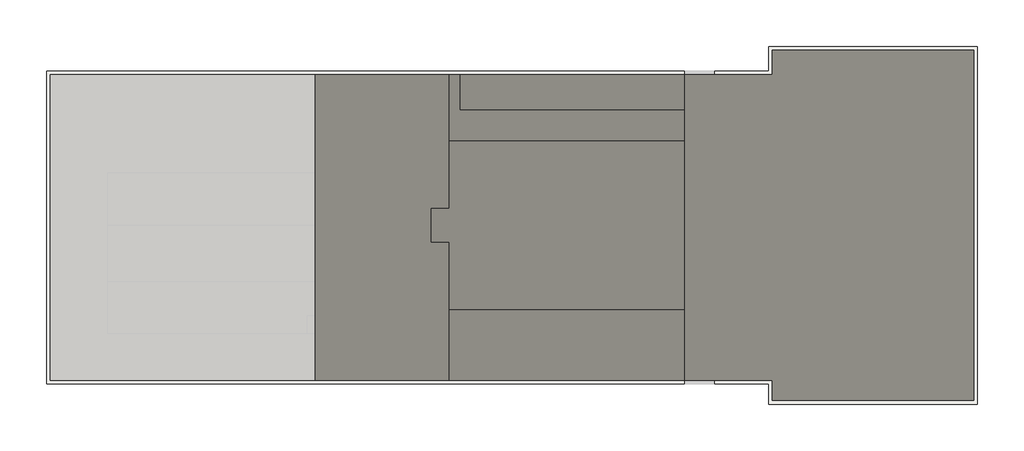
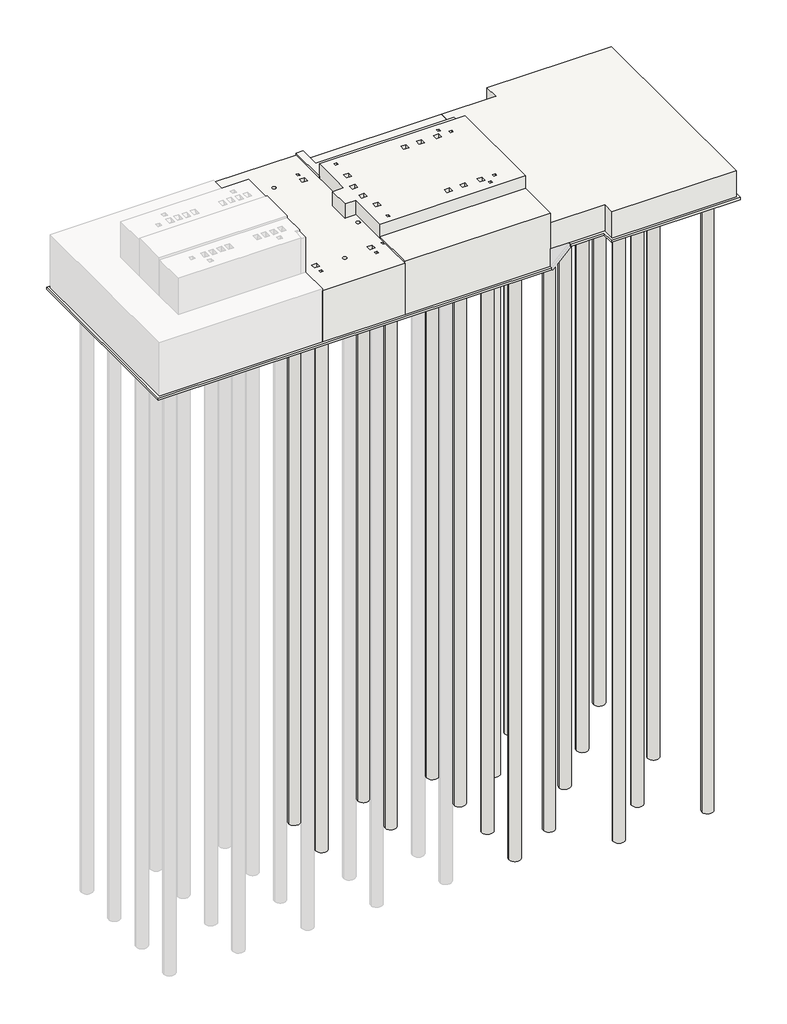
# One storey, part 2 of 2: 25 slabs.
"""IFC4 building model written with IfcOpenShell, lengths in millimetres."""

import ifcopenshell
import ifcopenshell.guid

model = None  # the IFC model being written
_history = None  # IfcOwnerHistory: only IFC2X3 demands one
_inside = {}  # id of a spatial element -> (the spatial element, [elements in it])
_under = {}  # id of a project, library or spatial element -> (it, [spatial elements below it])
_declared = {}  # id of a project -> (the project, [libraries it declares])
_typed = {}  # id of a type object -> (the type object, [elements of that type])
_made_of = {}  # id of a material, layer set ... -> (it, [elements and type objects made of it])


def new_model(schema):
    """Start an empty IFC model of exactly this schema.

    Asked for "IFC4X3", IfcOpenShell would pick the latest addendum, in which some entities
    have other attributes; the version numbers below select the first issue.
    IFC2X3 requires an IfcOwnerHistory on every rooted entity: one is made here for all.
    """
    global model, _history
    if schema == "IFC4X3":
        model = ifcopenshell.file(schema_version=(4, 3, 0, 0))
    else:
        model = ifcopenshell.file(schema=schema)
    _inside.clear()
    _under.clear()
    _declared.clear()
    _typed.clear()
    _made_of.clear()
    _history = None
    if model.schema == "IFC2X3":
        org = make("IfcOrganization", Name="unknown")
        user = make(
            "IfcPersonAndOrganization",
            ThePerson=make("IfcPerson", FamilyName="unknown"),
            TheOrganization=org,
        )
        app = make(
            "IfcApplication",
            ApplicationDeveloper=org,
            Version="unknown",
            ApplicationFullName="unknown",
            ApplicationIdentifier="unknown",
        )
        _history = make(
            "IfcOwnerHistory",
            OwningUser=user,
            OwningApplication=app,
            ChangeAction="ADDED",
            CreationDate=0,
        )
    return model


def make(cls, **values):
    """One entity of the class cls with the attributes given. An attribute that is None is left unset."""
    return model.create_entity(
        cls, **{name: value for name, value in values.items() if value is not None}
    )


def rooted(cls, **values):
    """An entity with a GlobalId (a new one), such as an element, a storey or a relation."""
    return make(cls, GlobalId=ifcopenshell.guid.new(), OwnerHistory=_history, **values)


def si_unit(unit_type, name, prefix=None):
    """IfcSIUnit, for example si_unit("LENGTHUNIT", "METRE", prefix="MILLI")."""
    return make("IfcSIUnit", UnitType=unit_type, Prefix=prefix, Name=name)


def assignment(units):
    """IfcUnitAssignment: the units of a project."""
    return None if units is None else make("IfcUnitAssignment", Units=units)


def point(xyz):
    """IfcCartesianPoint."""
    return None if xyz is None else make("IfcCartesianPoint", Coordinates=xyz)


def direction(xyz):
    """IfcDirection."""
    return None if xyz is None else make("IfcDirection", DirectionRatios=xyz)


def frame(location, z_axis=None, x_axis=None):
    """IfcAxis2Placement3D, a coordinate frame: its origin and axes. An axis left out is left unset."""
    return make(
        "IfcAxis2Placement3D",
        Location=point(location),
        Axis=direction(z_axis),
        RefDirection=direction(x_axis),
    )


def frame_2d(location, x_axis=None):
    """IfcAxis2Placement2D, a coordinate frame in the plane: its origin and x axis."""
    return make(
        "IfcAxis2Placement2D", Location=point(location), RefDirection=direction(x_axis)
    )


def origin():
    """The frame at (0, 0, 0) with its axes left unset."""
    return frame((0.0, 0.0, 0.0))


def place(relative_to, where):
    """IfcLocalPlacement: puts the frame where relative to a parent placement (None: the world)."""
    return make(
        "IfcLocalPlacement", PlacementRelTo=relative_to, RelativePlacement=where
    )


def context(
    kind, dimensions, precision=None, world=None, true_north=None, identifier=None
):
    """IfcGeometricRepresentationContext, for example the 3D "Model" context."""
    return make(
        "IfcGeometricRepresentationContext",
        ContextIdentifier=identifier,
        ContextType=kind,
        CoordinateSpaceDimension=dimensions,
        Precision=precision,
        WorldCoordinateSystem=world,
        TrueNorth=true_north,
    )


def project(units=None, contexts=None):
    """IfcProject with its units and contexts."""
    return rooted(
        "IfcProject",
        Name="project",
        RepresentationContexts=contexts,
        UnitsInContext=assignment(units),
    )


def spatial(cls, under=None, at=None, **own):
    """A site, building, storey or space (cls), placed at a placement, below another one or the project."""
    s = rooted(cls, ObjectPlacement=at, **own)
    if under is not None:
        _under.setdefault(under.id(), (under, []))[1].append(s)
    return s


def polyline(points):
    """IfcPolyline through the points."""
    return make("IfcPolyline", Points=[point(p) for p in points])


def circle_curve(where, radius):
    """IfcCircle in the frame where."""
    return make("IfcCircle", Position=where, Radius=radius)


def trimmed(basis, trim1, trim2, sense, master):
    """IfcTrimmedCurve: the piece of a basis curve between two trims."""
    return make(
        "IfcTrimmedCurve",
        BasisCurve=basis,
        Trim1=trim1,
        Trim2=trim2,
        SenseAgreement=sense,
        MasterRepresentation=master,
    )


def segment(curve, same_sense, transition):
    """IfcCompositeCurveSegment."""
    return make(
        "IfcCompositeCurveSegment",
        Transition=transition,
        SameSense=same_sense,
        ParentCurve=curve,
    )


def composite_curve(segments, self_intersect=None):
    """IfcCompositeCurve: segments joined end to end."""
    return make("IfcCompositeCurve", Segments=segments, SelfIntersect=self_intersect)


def outline(outer, holes=None, kind="AREA"):
    """IfcArbitraryClosedProfileDef: a profile drawn as a closed curve; with holes, ...WithVoids."""
    if holes is None:
        return make("IfcArbitraryClosedProfileDef", ProfileType=kind, OuterCurve=outer)
    return make(
        "IfcArbitraryProfileDefWithVoids",
        ProfileType=kind,
        OuterCurve=outer,
        InnerCurves=holes,
    )


def extrude(swept, where, along, depth):
    """IfcExtrudedAreaSolid: the profile swept, set in the frame where, extruded along a direction by depth."""
    return make(
        "IfcExtrudedAreaSolid",
        SweptArea=swept,
        Position=where,
        ExtrudedDirection=direction(along),
        Depth=depth,
    )


def faces_of(points, faces, orient=None, outer=None):
    """IfcFace entities. A face is a list of loops; a loop is a list of indices into points, from 0.

    orient and outer hold one flag for each loop. By default every Orientation is true, the
    first loop of a face is its IfcFaceOuterBound and the others are IfcFaceBound.
    """
    made = []
    for i, loops in enumerate(faces):
        bounds = []
        for j, loop in enumerate(loops):
            is_outer = j == 0 if outer is None else outer[i][j]
            bounds.append(
                make(
                    "IfcFaceOuterBound" if is_outer else "IfcFaceBound",
                    Bound=make("IfcPolyLoop", Polygon=[points[k] for k in loop]),
                    Orientation=True if orient is None else orient[i][j],
                )
            )
        made.append(make("IfcFace", Bounds=bounds))
    return made


def faceted_brep(points, faces, orient=None, outer=None, voids=None):
    """IfcFacetedBrep: a solid bounded by flat faces; with voids (closed shells), ...WithVoids."""
    shared = [point(p) for p in points]
    hull = make("IfcClosedShell", CfsFaces=faces_of(shared, faces, orient, outer))
    if voids is None:
        return make("IfcFacetedBrep", Outer=hull)
    return make(
        "IfcFacetedBrepWithVoids",
        Outer=hull,
        Voids=[
            make(cls, CfsFaces=faces_of(shared, fs, o, b)) for cls, fs, o, b in voids
        ],
    )


def shape(context_of_items, identifier, shape_type, items):
    """IfcShapeRepresentation: the items that make up one representation, for example the "Body"."""
    return make(
        "IfcShapeRepresentation",
        ContextOfItems=context_of_items,
        RepresentationIdentifier=identifier,
        RepresentationType=shape_type,
        Items=items,
    )


def made_of(thing, what):
    """Note that an element or type object is made of a material, layer set ...; save() writes the relation."""
    if what is not None:
        _made_of.setdefault(what.id(), (what, []))[1].append(thing)
    return thing


def element(
    cls,
    number,
    at=None,
    inside=None,
    cuts=None,
    type_object=None,
    material=None,
    context=None,
    identifier="Body",
    shape_type=None,
    held_by="IfcProductDefinitionShape",
    body=None,
    shapes=None,
    **own,
):
    """One element of the class cls, such as IfcWall. Its Tag is "e" and its number.

    at: its placement. inside: the storey or other place that contains it. cuts: it is an
    opening in that element (IfcRelVoidsElement). A single representation is given by context,
    identifier, shape_type and body (its items); several are given by shapes. held_by: the class
    of the entity that holds the representations. save() writes the other relations.
    """
    e = rooted(cls, Tag="e%d" % number, ObjectPlacement=at, **own)
    if body is not None:
        shapes = [shape(context, identifier, shape_type, body)]
    if shapes is not None:
        e.Representation = make(held_by, Representations=shapes)
    if inside is not None:
        _inside.setdefault(inside.id(), (inside, []))[1].append(e)
    if cuts is not None:
        rooted(
            "IfcRelVoidsElement", RelatingBuildingElement=cuts, RelatedOpeningElement=e
        )
    if type_object is not None:
        _typed.setdefault(type_object.id(), (type_object, []))[1].append(e)
    return made_of(e, material)


def aggregate(whole, parts):
    """IfcRelAggregates: a whole, such as a stair, and the parts it consists of."""
    return rooted("IfcRelAggregates", RelatingObject=whole, RelatedObjects=parts)


def save(model, path):
    """Write the relations noted so far, then the file.

    IfcRelAggregates (storeys below a building ...), IfcRelContainedInSpatialStructure (elements
    in a storey), IfcRelDefinesByType, IfcRelAssociatesMaterial and IfcRelDeclares: one each for
    every whole, place, type object, material and project.
    """
    for whole, parts in _under.values():
        aggregate(whole, parts)
    for where, things in _inside.values():
        rooted(
            "IfcRelContainedInSpatialStructure",
            RelatedElements=things,
            RelatingStructure=where,
        )
    for kind, things in _typed.values():
        rooted("IfcRelDefinesByType", RelatedObjects=things, RelatingType=kind)
    for what, things in _made_of.values():
        rooted("IfcRelAssociatesMaterial", RelatedObjects=things, RelatingMaterial=what)
    for by, libraries in _declared.values():
        rooted("IfcRelDeclares", RelatingContext=by, RelatedDefinitions=libraries)
    model.write(path)


def plane_surface(at):
    """IfcPlane: the flat surface through the origin of the frame at, square to its z axis."""
    return make("IfcPlane", Position=at)


def revolved_surface(curve, axis_point, axis_direction):
    """IfcSurfaceOfRevolution: the curve turned about the line through axis_point along axis_direction."""
    return make(
        "IfcSurfaceOfRevolution",
        SweptCurve=make("IfcArbitraryOpenProfileDef", ProfileType="CURVE", Curve=curve),
        AxisPosition=make("IfcAxis1Placement", Location=point(axis_point), Axis=direction(axis_direction)),
    )


def advanced_brep(points, edges, surfaces, faces):
    """IfcAdvancedBrep: a solid bounded by faces that lie on surfaces and meet in shared edges.

    An edge is (start, end): straight between two places in points (the first is 0);
    or (start, end, curve); or (start, end, curve, False) where it runs against its curve.
    A face is (place in surfaces, loops), or (place, loops, False) where it looks against
    its surface's normal. A loop lists edges by number (the first is 1), with a minus sign
    where the edge is run from its end to its start. The first loop is the outer one.
    """
    corners = [point(p) for p in points]
    vertices = [make("IfcVertexPoint", VertexGeometry=c) for c in corners]
    made = []
    for start, end, *more in edges:
        made.append(
            make(
                "IfcEdgeCurve",
                EdgeStart=vertices[start],
                EdgeEnd=vertices[end],
                EdgeGeometry=more[0] if more else make("IfcPolyline", Points=[corners[start], corners[end]]),
                SameSense=more[1] if len(more) > 1 else True,
            )
        )
    hull = []
    for where, loops, *sense in faces:
        bounds = []
        for j, loop in enumerate(loops):
            ring = [make("IfcOrientedEdge", EdgeElement=made[abs(k) - 1], Orientation=k > 0) for k in loop]
            bounds.append(
                make(
                    "IfcFaceOuterBound" if j == 0 else "IfcFaceBound",
                    Bound=make("IfcEdgeLoop", EdgeList=ring),
                    Orientation=True,
                )
            )
        hull.append(make("IfcAdvancedFace", Bounds=bounds, FaceSurface=surfaces[where], SameSense=sense[0] if sense else True))
    return make("IfcAdvancedBrep", Outer=make("IfcClosedShell", CfsFaces=hull))


model = new_model("IFC4")

# Units and contexts
model_context = context("Model", 3, world=origin())
ifc_project = project(units=[si_unit("LENGTHUNIT", "METRE", prefix="MILLI")], contexts=[model_context])

# Site, building, storey
site = spatial("IfcSite", under=ifc_project)
building = spatial("IfcBuilding", under=site)
storey = spatial("IfcBuildingStorey", under=building, Name="B.O.F", Elevation=2800.0)

# Slabs
placement = place(None, origin())
element("IfcSlab", 1, at=placement, inside=storey, context=model_context, shape_type="Brep", body=[
    faceted_brep([(10985.0, -7846.5096992, 2800.0), (10985.0, -8796.5096992, 2800.0), (17000.0, -8796.5096992, 2800.0), (17000.0, -9611.5096992, 2800.0), (10685.0, -9611.5096992, 2800.0), (10685.0, -7846.5096992, 2800.0), (10985.0, -7846.5096992, 5240.0), (10685.0, -7846.5096992, 5240.0), (10685.0, -9611.5096992, 5240.0), (17000.0, -9611.5096992, 5240.0), (17000.0, -8796.5096992, 5240.0), (10985.0, -8796.5096992, 5240.0), (10985.0, -7846.5096992, 4800.0), (10985.0, -8796.5096992, 4800.0), (17000.0, -8796.5096992, 4800.0), (10685.0, -7846.5096992, 5150.0)], [[[0, 1, 2, 3, 4, 5]], [[6, 7, 8, 9, 10, 11]], [[1, 0, 12, 6, 11, 13]], [[2, 1, 13, 11, 10, 14]], [[3, 2, 14, 10, 9]], [[4, 3, 9, 8]], [[5, 4, 8, 7, 15]], [[0, 5, 15, 7, 6, 12]]]),
    faceted_brep([(17000.0, -14161.5096992, 2800.0), (17000.0, -16046.5096992, 2800.0), (10685.0, -16046.5096992, 2800.0), (10685.0, -14161.5096992, 2800.0), (17000.0, -14161.5096992, 5240.0), (10685.0, -14161.5096992, 5240.0), (10685.0, -16046.5096992, 5240.0), (17000.0, -16046.5096992, 5240.0), (17000.0, -16046.5096992, 4800.0), (17000.0, -16046.5096992, 3600.0), (10685.0, -16046.5096992, 5150.0)], [[[0, 1, 2, 3]], [[4, 5, 6, 7]], [[1, 0, 4, 7, 8, 9]], [[2, 1, 9, 8, 7, 6, 10]], [[3, 2, 10, 6, 5]], [[0, 3, 5, 4]]]),
])
element("IfcSlab", 2, at=placement, inside=storey, context=model_context, shape_type="Brep", body=[
    faceted_brep([(17000.0, -7846.5096992, 2800.0), (17000.0, -8796.5096992, 2800.0), (10985.0, -8796.5096992, 2800.0), (10985.0, -7846.5096992, 2800.0), (17000.0, -8796.5096992, 4800.0), (17000.0, -7846.5096992, 4800.0), (10985.0, -7846.5096992, 4800.0), (10985.0, -8796.5096992, 4800.0), (17000.0, -7846.5096992, 3600.0)], [[[0, 1, 2, 3]], [[4, 5, 6, 7]], [[1, 0, 8, 5, 4]], [[2, 1, 4, 7]], [[3, 2, 7, 6]], [[0, 3, 6, 5, 8]]]),
])
element("IfcSlab", 3, at=placement, inside=storey, context=model_context, shape_type="Brep", body=[
    faceted_brep([(10685.0, -11426.4596992, 2800.0), (10685.0, -9611.5096992, 2800.0), (17000.0, -9611.5096992, 2800.0), (17000.0, -14161.5096992, 2800.0), (10685.0, -14161.5096992, 2800.0), (10685.0, -12346.4596992, 2800.0), (10200.0, -12346.4596992, 2800.0), (10200.0, -11426.4596992, 2800.0), (10685.0, -9611.5096992, 5810.0), (10685.0, -11426.4596992, 5810.0), (10200.0, -11426.4596992, 5810.0), (10200.0, -12346.4596992, 5810.0), (10685.0, -12346.4596992, 5810.0), (10685.0, -14161.5096992, 5810.0), (17000.0, -14161.5096992, 5810.0), (17000.0, -9611.5096992, 5810.0), (11330.0, -12876.5096992, 5810.0), (11330.0, -13096.5096992, 5810.0), (11110.0, -13096.5096992, 5810.0), (11110.0, -12876.5096992, 5810.0), (11165.0, -9876.5096992, 5810.0), (11275.0, -9876.5096992, 5810.0), (11275.0, -9986.5096992, 5810.0), (11165.0, -9986.5096992, 5810.0), (15600.0, -9876.5096992, 5810.0), (15710.0, -9876.5096992, 5810.0), (15710.0, -9986.5096992, 5810.0), (15600.0, -9986.5096992, 5810.0), (15975.0, -10196.5096992, 5810.0), (16085.0, -10196.5096992, 5810.0), (16085.0, -10306.5096992, 5810.0), (15975.0, -10306.5096992, 5810.0), (15600.0, -13786.5096992, 5810.0), (15710.0, -13786.5096992, 5810.0), (15710.0, -13896.5096992, 5810.0), (15600.0, -13896.5096992, 5810.0), (15975.0, -13466.5096992, 5810.0), (16085.0, -13466.5096992, 5810.0), (16085.0, -13576.5096992, 5810.0), (15975.0, -13576.5096992, 5810.0), (11165.0, -13786.5096992, 5810.0), (11275.0, -13786.5096992, 5810.0), (11275.0, -13896.5096992, 5810.0), (11165.0, -13896.5096992, 5810.0), (11160.0, -12116.5096992, 5810.0), (11160.0, -12336.5096992, 5810.0), (10940.0, -12336.5096992, 5810.0), (10940.0, -12116.5096992, 5810.0), (11160.0, -11436.5096992, 5810.0), (11160.0, -11656.5096992, 5810.0), (10940.0, -11656.5096992, 5810.0), (10940.0, -11436.5096992, 5810.0), (11330.0, -10676.5096992, 5810.0), (11330.0, -10896.5096992, 5810.0), (11110.0, -10896.5096992, 5810.0), (11110.0, -10676.5096992, 5810.0), (14795.0, -10141.5096992, 5810.0), (14795.0, -10361.5096992, 5810.0), (14575.0, -10361.5096992, 5810.0), (14575.0, -10141.5096992, 5810.0), (15540.0, -10141.5096992, 5810.0), (15540.0, -10361.5096992, 5810.0), (15320.0, -10361.5096992, 5810.0), (15320.0, -10141.5096992, 5810.0), (14125.0, -13411.4096992, 5810.0), (14125.0, -13631.4096992, 5810.0), (13905.0, -13631.4096992, 5810.0), (13905.0, -13411.4096992, 5810.0), (14795.0, -13411.4096992, 5810.0), (14795.0, -13631.4096992, 5810.0), (14575.0, -13631.4096992, 5810.0), (14575.0, -13411.4096992, 5810.0), (15540.0, -13411.4096992, 5810.0), (15540.0, -13631.4096992, 5810.0), (15320.0, -13631.4096992, 5810.0), (15320.0, -13411.4096992, 5810.0), (14125.0, -10141.5096992, 5810.0), (14125.0, -10361.5096992, 5810.0), (13905.0, -10361.5096992, 5810.0), (13905.0, -10141.5096992, 5810.0), (10685.0, -11426.4596992, 5150.0), (10685.0, -9611.5096992, 5240.0), (17000.0, -9611.5096992, 5240.0), (17000.0, -14161.5096992, 5240.0), (10685.0, -14161.5096992, 5240.0), (10685.0, -12346.4596992, 5150.0), (10200.0, -12346.4596992, 5150.0), (10200.0, -11426.4596992, 5150.0), (11380.0, -12826.5096992, 4960.0), (11060.0, -12826.5096992, 4960.0), (11060.0, -13146.5096992, 4960.0), (11380.0, -13146.5096992, 4960.0), (11275.0, -9876.5096992, 5609.9618634), (11165.0, -9876.5096992, 5609.9618634), (11165.0, -9986.5096992, 5609.9618634), (11275.0, -9986.5096992, 5609.9618634), (15710.0, -9876.5096992, 5609.9618634), (15600.0, -9876.5096992, 5609.9618634), (15600.0, -9986.5096992, 5609.9618634), (15710.0, -9986.5096992, 5609.9618634), (16085.0, -10196.5096992, 5609.9618634), (15975.0, -10196.5096992, 5609.9618634), (15975.0, -10306.5096992, 5609.9618634), (16085.0, -10306.5096992, 5609.9618634), (15710.0, -13786.5096992, 5609.9618634), (15600.0, -13786.5096992, 5609.9618634), (15600.0, -13896.5096992, 5609.9618634), (15710.0, -13896.5096992, 5609.9618634), (16085.0, -13466.5096992, 5609.9618634), (15975.0, -13466.5096992, 5609.9618634), (15975.0, -13576.5096992, 5609.9618634), (16085.0, -13576.5096992, 5609.9618634), (11275.0, -13786.5096992, 5609.9618634), (11165.0, -13786.5096992, 5609.9618634), (11165.0, -13896.5096992, 5609.9618634), (11275.0, -13896.5096992, 5609.9618634), (11210.0, -12066.5096992, 4960.0), (10890.0, -12066.5096992, 4960.0), (10890.0, -12386.5096992, 4960.0), (11210.0, -12386.5096992, 4960.0), (11210.0, -11386.5096992, 4960.0), (10890.0, -11386.5096992, 4960.0), (10890.0, -11706.5096992, 4960.0), (11210.0, -11706.5096992, 4960.0), (11380.0, -10626.5096992, 4960.0), (11060.0, -10626.5096992, 4960.0), (11060.0, -10946.5096992, 4960.0), (11380.0, -10946.5096992, 4960.0), (14845.0, -10091.5096992, 4960.0), (14525.0, -10091.5096992, 4960.0), (14525.0, -10411.5096992, 4960.0), (14845.0, -10411.5096992, 4960.0), (15590.0, -10091.5096992, 4960.0), (15270.0, -10091.5096992, 4960.0), (15270.0, -10411.5096992, 4960.0), (15590.0, -10411.5096992, 4960.0), (14175.0, -13361.4096992, 4960.0), (13855.0, -13361.4096992, 4960.0), (13855.0, -13681.4096992, 4960.0), (14175.0, -13681.4096992, 4960.0), (14845.0, -13361.4096992, 4960.0), (14525.0, -13361.4096992, 4960.0), (14525.0, -13681.4096992, 4960.0), (14845.0, -13681.4096992, 4960.0), (15590.0, -13361.4096992, 4960.0), (15270.0, -13361.4096992, 4960.0), (15270.0, -13681.4096992, 4960.0), (15590.0, -13681.4096992, 4960.0), (14175.0, -10091.5096992, 4960.0), (13855.0, -10091.5096992, 4960.0), (13855.0, -10411.5096992, 4960.0), (14175.0, -10411.5096992, 4960.0)], [[[0, 1, 2, 3, 4, 5, 6, 7]], [[8, 9, 10, 11, 12, 13, 14, 15], [16, 17, 18, 19], [20, 21, 22, 23], [24, 25, 26, 27], [28, 29, 30, 31], [32, 33, 34, 35], [36, 37, 38, 39], [40, 41, 42, 43], [44, 45, 46, 47], [48, 49, 50, 51], [52, 53, 54, 55], [56, 57, 58, 59], [60, 61, 62, 63], [64, 65, 66, 67], [68, 69, 70, 71], [72, 73, 74, 75], [76, 77, 78, 79]], [[1, 0, 80, 9, 8, 81]], [[2, 1, 81, 8, 15, 82]], [[3, 2, 82, 15, 14, 83]], [[4, 3, 83, 14, 13, 84]], [[5, 4, 84, 13, 12, 85]], [[6, 5, 85, 12, 11, 86]], [[7, 6, 86, 11, 10, 87]], [[0, 7, 87, 10, 9, 80]], [[88, 89, 90, 91]], [[88, 91, 17, 16]], [[91, 90, 18, 17]], [[90, 89, 19, 18]], [[89, 88, 16, 19]], [[92, 93, 94, 95]], [[93, 92, 21, 20]], [[94, 93, 20, 23]], [[95, 94, 23, 22]], [[92, 95, 22, 21]], [[96, 97, 98, 99]], [[100, 101, 102, 103]], [[104, 105, 106, 107]], [[108, 109, 110, 111]], [[97, 96, 25, 24]], [[98, 97, 24, 27]], [[99, 98, 27, 26]], [[96, 99, 26, 25]], [[101, 100, 29, 28]], [[102, 101, 28, 31]], [[103, 102, 31, 30]], [[100, 103, 30, 29]], [[105, 104, 33, 32]], [[106, 105, 32, 35]], [[107, 106, 35, 34]], [[104, 107, 34, 33]], [[109, 108, 37, 36]], [[110, 109, 36, 39]], [[111, 110, 39, 38]], [[108, 111, 38, 37]], [[112, 113, 114, 115]], [[113, 112, 41, 40]], [[114, 113, 40, 43]], [[115, 114, 43, 42]], [[112, 115, 42, 41]], [[116, 117, 118, 119]], [[116, 119, 45, 44]], [[119, 118, 46, 45]], [[118, 117, 47, 46]], [[117, 116, 44, 47]], [[120, 121, 122, 123]], [[120, 123, 49, 48]], [[123, 122, 50, 49]], [[122, 121, 51, 50]], [[121, 120, 48, 51]], [[124, 125, 126, 127]], [[124, 127, 53, 52]], [[127, 126, 54, 53]], [[126, 125, 55, 54]], [[125, 124, 52, 55]], [[128, 129, 130, 131]], [[128, 131, 57, 56]], [[131, 130, 58, 57]], [[130, 129, 59, 58]], [[129, 128, 56, 59]], [[132, 133, 134, 135]], [[132, 135, 61, 60]], [[135, 134, 62, 61]], [[134, 133, 63, 62]], [[133, 132, 60, 63]], [[136, 137, 138, 139]], [[136, 139, 65, 64]], [[139, 138, 66, 65]], [[138, 137, 67, 66]], [[137, 136, 64, 67]], [[140, 141, 142, 143]], [[140, 143, 69, 68]], [[143, 142, 70, 69]], [[142, 141, 71, 70]], [[141, 140, 68, 71]], [[144, 145, 146, 147]], [[144, 147, 73, 72]], [[147, 146, 74, 73]], [[146, 145, 75, 74]], [[145, 144, 72, 75]], [[148, 149, 150, 151]], [[148, 151, 77, 76]], [[151, 150, 78, 77]], [[150, 149, 79, 78]], [[149, 148, 76, 79]]]),
])
element("IfcSlab", 4, at=placement, inside=storey, context=model_context, shape_type="AdvancedBrep", body=[
    advanced_brep(
    [(10685.0, -11426.4596992, 2800.0), (10200.0, -11426.4596992, 2800.0), (10200.0, -12346.4596992, 2800.0), (10685.0, -12346.4596992, 2800.0), (10685.0, -14161.5096992, 2800.0), (10685.0, -16046.5096992, 2800.0), (7095.0, -16046.5096992, 2800.0), (7095.0, -14786.5096992, 2800.0), (7095.0, -14316.5096992, 2800.0), (7095.0, -13386.5096992, 2800.0), (7095.0, -11886.5096992, 2800.0), (7095.0, -10486.5096992, 2800.0), (7095.0, -7846.5096992, 2800.0), (10685.0, -7846.5096992, 2800.0), (10685.0, -9611.5096992, 2800.0), (10200.0, -11426.4596992, 5150.0), (10685.0, -11426.4596992, 5150.0), (10685.0, -9611.5096992, 5150.0), (10685.0, -7846.5096992, 5150.0), (7095.0, -7846.5096992, 5150.0), (7095.0, -9346.5096992, 5150.0), (7205.0, -9346.5096992, 5150.0), (7205.0, -9456.5096992, 5150.0), (7095.0, -9456.5096992, 5150.0), (7095.0, -16046.5096992, 5150.0), (10685.0, -16046.5096992, 5150.0), (10685.0, -14546.5096992, 5150.0), (10575.0, -14546.5096992, 5150.0), (10575.0, -14436.5096992, 5150.0), (10685.0, -14436.5096992, 5150.0), (10685.0, -14161.5096992, 5150.0), (10685.0, -12346.4596992, 5150.0), (10200.0, -12346.4596992, 5150.0), (8975.0, -9291.5096992, 5150.0), (8815.0, -9291.5096992, 5150.0), (7370.0, -12831.5096992, 5150.0), (7210.0, -12831.5096992, 5150.0), (8975.0, -14601.5096992, 5150.0), (8815.0, -14601.5096992, 5150.0), (10580.0, -12831.5096992, 5150.0), (10420.0, -12831.5096992, 5150.0), (7635.0, -8946.5096992, 5150.0), (7745.0, -8946.5096992, 5150.0), (7745.0, -9056.5096992, 5150.0), (7635.0, -9056.5096992, 5150.0), (10045.0, -8946.5096992, 5150.0), (10155.0, -8946.5096992, 5150.0), (10155.0, -9056.5096992, 5150.0), (10045.0, -9056.5096992, 5150.0), (7635.0, -14836.5096992, 5150.0), (7745.0, -14836.5096992, 5150.0), (7745.0, -14946.5096992, 5150.0), (7635.0, -14946.5096992, 5150.0), (10045.0, -14836.5096992, 5150.0), (10155.0, -14836.5096992, 5150.0), (10155.0, -14946.5096992, 5150.0), (10045.0, -14946.5096992, 5150.0), (7800.0, -14381.5096992, 5150.0), (7800.0, -14601.5096992, 5150.0), (7580.0, -14601.5096992, 5150.0), (7580.0, -14381.5096992, 5150.0), (10210.0, -14381.5096992, 5150.0), (10210.0, -14601.5096992, 5150.0), (9990.0, -14601.5096992, 5150.0), (9990.0, -14381.5096992, 5150.0), (10210.0, -9291.5096992, 5150.0), (10210.0, -9511.5096992, 5150.0), (9990.0, -9511.5096992, 5150.0), (9990.0, -9291.5096992, 5150.0), (7800.0, -9291.5096992, 5150.0), (7800.0, -9511.5096992, 5150.0), (7580.0, -9511.5096992, 5150.0), (7580.0, -9291.5096992, 5150.0), (10685.0, -14436.5096992, 4949.9618634), (10685.0, -14546.5096992, 4949.9618634), (7095.0, -9456.5096992, 4949.9618634), (7095.0, -9346.5096992, 4949.9618634), (8815.0, -9291.5096992, 4949.9618634), (8975.0, -9291.5096992, 4949.9618634), (7210.0, -12831.5096992, 4849.9618634), (7370.0, -12831.5096992, 4849.9618634), (8815.0, -14601.5096992, 4849.9618634), (8975.0, -14601.5096992, 4849.9618634), (10420.0, -12831.5096992, 4849.9618634), (10580.0, -12831.5096992, 4849.9618634), (7745.0, -8946.5096992, 4949.9618634), (7635.0, -8946.5096992, 4949.9618634), (7635.0, -9056.5096992, 4949.9618634), (7745.0, -9056.5096992, 4949.9618634), (7205.0, -9346.5096992, 4949.9618634), (7205.0, -9456.5096992, 4949.9618634), (10155.0, -8946.5096992, 4949.9618634), (10045.0, -8946.5096992, 4949.9618634), (10045.0, -9056.5096992, 4949.9618634), (10155.0, -9056.5096992, 4949.9618634), (7745.0, -14836.5096992, 4949.9618634), (7635.0, -14836.5096992, 4949.9618634), (7635.0, -14946.5096992, 4949.9618634), (7745.0, -14946.5096992, 4949.9618634), (10155.0, -14836.5096992, 4949.9618634), (10045.0, -14836.5096992, 4949.9618634), (10045.0, -14946.5096992, 4949.9618634), (10155.0, -14946.5096992, 4949.9618634), (10575.0, -14436.5096992, 4949.9618634), (10575.0, -14546.5096992, 4949.9618634), (7850.0, -14331.5096992, 4300.0), (7530.0, -14331.5096992, 4300.0), (7530.0, -14651.5096992, 4300.0), (7850.0, -14651.5096992, 4300.0), (10260.0, -14331.5096992, 4300.0), (9940.0, -14331.5096992, 4300.0), (9940.0, -14651.5096992, 4300.0), (10260.0, -14651.5096992, 4300.0), (10260.0, -9241.5096992, 4300.0), (9940.0, -9241.5096992, 4300.0), (9940.0, -9561.5096992, 4300.0), (10260.0, -9561.5096992, 4300.0), (7850.0, -9241.5096992, 4300.0), (7530.0, -9241.5096992, 4300.0), (7530.0, -9561.5096992, 4300.0), (7850.0, -9561.5096992, 4300.0)],
    [
        (0, 1),
        (1, 2),
        (2, 3),
        (3, 4),
        (4, 5),
        (5, 6),
        (6, 7),
        (7, 8),
        (8, 9),
        (9, 10),
        (10, 11),
        (11, 12),
        (12, 13),
        (13, 14),
        (14, 0),
        (15, 16),
        (16, 17),
        (17, 18),
        (18, 19),
        (19, 20),
        (20, 21),
        (21, 22),
        (22, 23),
        (23, 24),
        (24, 25),
        (25, 26),
        (26, 27),
        (27, 28),
        (28, 29),
        (29, 30),
        (30, 31),
        (31, 32),
        (32, 15),
        (33, 34, circle_curve(frame((8895.0, -9291.5096992, 5150.0), z_axis=(0.0, 0.0, -1.0), x_axis=(1.0, 0.0, 0.0)), 80.0)),
        (34, 33, circle_curve(frame((8895.0, -9291.5096992, 5150.0), z_axis=(0.0, 0.0, -1.0), x_axis=(1.0, 0.0, 0.0)), 80.0)),
        (35, 36, circle_curve(frame((7290.0, -12831.5096992, 5150.0), z_axis=(0.0, 0.0, -1.0), x_axis=(1.0, 0.0, 0.0)), 80.0)),
        (36, 35, circle_curve(frame((7290.0, -12831.5096992, 5150.0), z_axis=(0.0, 0.0, -1.0), x_axis=(1.0, 0.0, 0.0)), 80.0)),
        (37, 38, circle_curve(frame((8895.0, -14601.5096992, 5150.0), z_axis=(0.0, 0.0, -1.0), x_axis=(1.0, 0.0, 0.0)), 80.0)),
        (38, 37, circle_curve(frame((8895.0, -14601.5096992, 5150.0), z_axis=(0.0, 0.0, -1.0), x_axis=(1.0, 0.0, 0.0)), 80.0)),
        (39, 40, circle_curve(frame((10500.0, -12831.5096992, 5150.0), z_axis=(0.0, 0.0, -1.0), x_axis=(1.0, 0.0, 0.0)), 80.0)),
        (40, 39, circle_curve(frame((10500.0, -12831.5096992, 5150.0), z_axis=(0.0, 0.0, -1.0), x_axis=(1.0, 0.0, 0.0)), 80.0)),
        (41, 42),
        (42, 43),
        (43, 44),
        (44, 41),
        (45, 46),
        (46, 47),
        (47, 48),
        (48, 45),
        (49, 50),
        (50, 51),
        (51, 52),
        (52, 49),
        (53, 54),
        (54, 55),
        (55, 56),
        (56, 53),
        (57, 58),
        (58, 59),
        (59, 60),
        (60, 57),
        (61, 62),
        (62, 63),
        (63, 64),
        (64, 61),
        (65, 66),
        (66, 67),
        (67, 68),
        (68, 65),
        (69, 70),
        (70, 71),
        (71, 72),
        (72, 69),
        (16, 0),
        (13, 18),
        (15, 1),
        (32, 2),
        (31, 3),
        (29, 73),
        (73, 74),
        (74, 26),
        (25, 5),
        (24, 6),
        (23, 75),
        (75, 76),
        (76, 20),
        (19, 12),
        (77, 78, circle_curve(frame((8895.0, -9291.5096992, 4949.9618634), z_axis=(0.0, 0.0, 1.0), x_axis=(1.0, 0.0, 0.0)), 80.0)),
        (78, 77, circle_curve(frame((8895.0, -9291.5096992, 4949.9618634), z_axis=(0.0, 0.0, 1.0), x_axis=(1.0, 0.0, 0.0)), 80.0)),
        (77, 34),
        (33, 78),
        (79, 80, circle_curve(frame((7290.0, -12831.5096992, 4849.9618634), z_axis=(0.0, 0.0, 1.0), x_axis=(1.0, 0.0, 0.0)), 80.0)),
        (80, 79, circle_curve(frame((7290.0, -12831.5096992, 4849.9618634), z_axis=(0.0, 0.0, 1.0), x_axis=(1.0, 0.0, 0.0)), 80.0)),
        (81, 82, circle_curve(frame((8895.0, -14601.5096992, 4849.9618634), z_axis=(0.0, 0.0, 1.0), x_axis=(1.0, 0.0, 0.0)), 80.0)),
        (82, 81, circle_curve(frame((8895.0, -14601.5096992, 4849.9618634), z_axis=(0.0, 0.0, 1.0), x_axis=(1.0, 0.0, 0.0)), 80.0)),
        (83, 84, circle_curve(frame((10500.0, -12831.5096992, 4849.9618634), z_axis=(0.0, 0.0, 1.0), x_axis=(1.0, 0.0, 0.0)), 80.0)),
        (84, 83, circle_curve(frame((10500.0, -12831.5096992, 4849.9618634), z_axis=(0.0, 0.0, 1.0), x_axis=(1.0, 0.0, 0.0)), 80.0)),
        (79, 36),
        (35, 80),
        (81, 38),
        (37, 82),
        (83, 40),
        (39, 84),
        (85, 86),
        (86, 87),
        (87, 88),
        (88, 85),
        (89, 76),
        (75, 90),
        (90, 89),
        (91, 92),
        (92, 93),
        (93, 94),
        (94, 91),
        (95, 96),
        (96, 97),
        (97, 98),
        (98, 95),
        (99, 100),
        (100, 101),
        (101, 102),
        (102, 99),
        (73, 103),
        (103, 104),
        (104, 74),
        (85, 42),
        (41, 86),
        (44, 87),
        (43, 88),
        (89, 21),
        (22, 90),
        (91, 46),
        (45, 92),
        (48, 93),
        (47, 94),
        (95, 50),
        (49, 96),
        (52, 97),
        (51, 98),
        (99, 54),
        (53, 100),
        (56, 101),
        (55, 102),
        (28, 103),
        (27, 104),
        (105, 106),
        (106, 107),
        (107, 108),
        (108, 105),
        (108, 58),
        (57, 105),
        (107, 59),
        (106, 60),
        (109, 110),
        (110, 111),
        (111, 112),
        (112, 109),
        (112, 62),
        (61, 109),
        (111, 63),
        (110, 64),
        (113, 114),
        (114, 115),
        (115, 116),
        (116, 113),
        (116, 66),
        (65, 113),
        (115, 67),
        (114, 68),
        (117, 118),
        (118, 119),
        (119, 120),
        (120, 117),
        (120, 70),
        (69, 117),
        (119, 71),
        (118, 72),
    ],
    [
        plane_surface(frame((10685.0, -7846.5096992, 2800.0), z_axis=(0.0, 0.0, -1.0), x_axis=(0.0, -1.0, 0.0))),
        plane_surface(frame((10685.0, -7846.5096992, 5150.0), z_axis=(0.0, 0.0, 1.0), x_axis=(0.0, 1.0, 0.0))),
        plane_surface(frame((10685.0, -7846.5096992, 2800.0), z_axis=(1.0, 0.0, 0.0), x_axis=(0.0, 0.0, 1.0))),
        plane_surface(frame((10685.0, -11426.4596992, 2800.0), z_axis=(0.0, -1.0, 0.0), x_axis=(0.0, 0.0, 1.0))),
        plane_surface(frame((10200.0, -11426.4596992, 2800.0), z_axis=(1.0, 0.0, 0.0), x_axis=(0.0, 0.0, 1.0))),
        plane_surface(frame((10200.0, -12346.4596992, 2800.0), z_axis=(0.0, 1.0, 0.0), x_axis=(0.0, 0.0, 1.0))),
        plane_surface(frame((10685.0, -12346.4596992, 2800.0), z_axis=(1.0, 0.0, 0.0), x_axis=(0.0, 0.0, 1.0))),
        plane_surface(frame((10685.0, -16046.5096992, 2800.0), z_axis=(0.0, -1.0, 0.0), x_axis=(0.0, 0.0, 1.0))),
        plane_surface(frame((7095.0, -16046.5096992, 2800.0), z_axis=(-1.0, 0.0, 0.0), x_axis=(0.0, 0.0, 1.0))),
        plane_surface(frame((7095.0, -7846.5096992, 2800.0), z_axis=(0.0, 1.0, 0.0), x_axis=(0.0, 0.0, 1.0))),
        plane_surface(frame((8975.0, -9291.5096992, 4949.9618634), z_axis=(0.0, 0.0, 1.0), x_axis=(0.0, -1.0, 0.0))),
        revolved_surface(polyline([(8975.0, -9291.5096992, 5150.0), (8975.0, -9291.5096992, 4949.9618634)]), (8895.0, -9291.5096992, 4949.9618634), (0.0, 0.0, 1.0)),
        plane_surface(frame((7370.0, -12831.5096992, 4849.9618634), z_axis=(0.0, 0.0, 1.0), x_axis=(0.0, -1.0, 0.0))),
        revolved_surface(polyline([(7370.0, -12831.5096992, 5150.0), (7370.0, -12831.5096992, 4849.9618634)]), (7290.0, -12831.5096992, 4849.9618634), (0.0, 0.0, 1.0)),
        revolved_surface(polyline([(8975.0, -14601.5096992, 5150.0), (8975.0, -14601.5096992, 4849.9618634)]), (8895.0, -14601.5096992, 4799.9618634), (0.0, 0.0, 1.0)),
        revolved_surface(polyline([(10580.0, -12831.5096992, 5150.0), (10580.0, -12831.5096992, 4849.9618634)]), (10500.0, -12831.5096992, 4799.9618634), (0.0, 0.0, 1.0)),
        plane_surface(frame((7635.0, -8946.5096992, 4949.9618634), z_axis=(0.0, 0.0, 1.0), x_axis=(1.0, 0.0, 0.0))),
        plane_surface(frame((7745.0, -8946.5096992, 5149.9618634), z_axis=(0.0, -1.0, 0.0), x_axis=(0.0, 0.0, -1.0))),
        plane_surface(frame((7635.0, -8946.5096992, 5149.9618634), z_axis=(1.0, 0.0, 0.0), x_axis=(0.0, 0.0, -1.0))),
        plane_surface(frame((7635.0, -9056.5096992, 5149.9618634), z_axis=(0.0, 1.0, 0.0), x_axis=(0.0, 0.0, -1.0))),
        plane_surface(frame((7745.0, -9056.5096992, 5149.9618634), z_axis=(-1.0, 0.0, 0.0), x_axis=(0.0, 0.0, -1.0))),
        plane_surface(frame((7205.0, -9346.5096992, 5149.9618634), z_axis=(0.0, -1.0, 0.0), x_axis=(0.0, 0.0, -1.0))),
        plane_surface(frame((7095.0, -9456.5096992, 5149.9618634), z_axis=(0.0, 1.0, 0.0), x_axis=(0.0, 0.0, -1.0))),
        plane_surface(frame((7205.0, -9456.5096992, 5149.9618634), z_axis=(-1.0, 0.0, 0.0), x_axis=(0.0, 0.0, -1.0))),
        plane_surface(frame((10155.0, -8946.5096992, 5149.9618634), z_axis=(0.0, -1.0, 0.0), x_axis=(0.0, 0.0, -1.0))),
        plane_surface(frame((10045.0, -8946.5096992, 5149.9618634), z_axis=(1.0, 0.0, 0.0), x_axis=(0.0, 0.0, -1.0))),
        plane_surface(frame((10045.0, -9056.5096992, 5149.9618634), z_axis=(0.0, 1.0, 0.0), x_axis=(0.0, 0.0, -1.0))),
        plane_surface(frame((10155.0, -9056.5096992, 5149.9618634), z_axis=(-1.0, 0.0, 0.0), x_axis=(0.0, 0.0, -1.0))),
        plane_surface(frame((7745.0, -14836.5096992, 5149.9618634), z_axis=(0.0, -1.0, 0.0), x_axis=(0.0, 0.0, -1.0))),
        plane_surface(frame((7635.0, -14836.5096992, 5149.9618634), z_axis=(1.0, 0.0, 0.0), x_axis=(0.0, 0.0, -1.0))),
        plane_surface(frame((7635.0, -14946.5096992, 5149.9618634), z_axis=(0.0, 1.0, 0.0), x_axis=(0.0, 0.0, -1.0))),
        plane_surface(frame((7745.0, -14946.5096992, 5149.9618634), z_axis=(-1.0, 0.0, 0.0), x_axis=(0.0, 0.0, -1.0))),
        plane_surface(frame((10155.0, -14836.5096992, 5149.9618634), z_axis=(0.0, -1.0, 0.0), x_axis=(0.0, 0.0, -1.0))),
        plane_surface(frame((10045.0, -14836.5096992, 5149.9618634), z_axis=(1.0, 0.0, 0.0), x_axis=(0.0, 0.0, -1.0))),
        plane_surface(frame((10045.0, -14946.5096992, 5149.9618634), z_axis=(0.0, 1.0, 0.0), x_axis=(0.0, 0.0, -1.0))),
        plane_surface(frame((10155.0, -14946.5096992, 5149.9618634), z_axis=(-1.0, 0.0, 0.0), x_axis=(0.0, 0.0, -1.0))),
        plane_surface(frame((10685.0, -14436.5096992, 5149.9618634), z_axis=(0.0, -1.0, 0.0), x_axis=(0.0, 0.0, -1.0))),
        plane_surface(frame((10575.0, -14436.5096992, 5149.9618634), z_axis=(1.0, 0.0, 0.0), x_axis=(0.0, 0.0, -1.0))),
        plane_surface(frame((10575.0, -14546.5096992, 5149.9618634), z_axis=(0.0, 1.0, 0.0), x_axis=(0.0, 0.0, -1.0))),
        plane_surface(frame((7690.0, -14491.5096992, 4300.0), z_axis=(0.0, 0.0, 1.0), x_axis=(0.0, -1.0, 0.0))),
        plane_surface(frame((7800.0, -14491.5096992, 5150.0), z_axis=(-0.998274373174996, 0.0, -0.05872202195146968), x_axis=(0.0, -1.0, 0.0))),
        plane_surface(frame((7690.0, -14601.5096992, 5150.0), z_axis=(0.0, 0.998274373174996, -0.058722021951469715), x_axis=(-1.0, 0.0, 0.0))),
        plane_surface(frame((7580.0, -14491.5096992, 5150.0), z_axis=(0.9982743731749959, 0.0, -0.05872202195147098), x_axis=(0.0, 1.0, 0.0))),
        plane_surface(frame((7690.0, -14381.5096992, 5150.0), z_axis=(0.0, -0.9982743731749959, -0.058722021951472254), x_axis=(1.0, 0.0, 0.0))),
        plane_surface(frame((10100.0, -14491.5096992, 4300.0), z_axis=(0.0, 0.0, 1.0), x_axis=(0.0, -1.0, 0.0))),
        plane_surface(frame((10210.0, -14491.5096992, 5150.0), z_axis=(-0.9982743731749959, 0.0, -0.05872202195147221), x_axis=(0.0, -1.0, 0.0))),
        plane_surface(frame((10100.0, -14601.5096992, 5150.0), z_axis=(0.0, 0.998274373174996, -0.058722021951469715), x_axis=(-1.0, 0.0, 0.0))),
        plane_surface(frame((9990.0, -14491.5096992, 5150.0), z_axis=(0.9982743731749959, 0.0, -0.058722021951472254), x_axis=(0.0, 1.0, 0.0))),
        plane_surface(frame((10100.0, -14381.5096992, 5150.0), z_axis=(0.0, -0.9982743731749959, -0.058722021951472254), x_axis=(1.0, 0.0, 0.0))),
        plane_surface(frame((10100.0, -9401.5096992, 4300.0), z_axis=(0.0, 0.0, 1.0), x_axis=(0.0, -1.0, 0.0))),
        plane_surface(frame((10210.0, -9401.5096992, 5150.0), z_axis=(-0.9982743731749959, 0.0, -0.05872202195147221), x_axis=(0.0, -1.0, 0.0))),
        plane_surface(frame((10100.0, -9511.5096992, 5150.0), z_axis=(0.0, 0.998274373174996, -0.058722021951469715), x_axis=(-1.0, 0.0, 0.0))),
        plane_surface(frame((9990.0, -9401.5096992, 5150.0), z_axis=(0.9982743731749959, 0.0, -0.058722021951472254), x_axis=(0.0, 1.0, 0.0))),
        plane_surface(frame((10100.0, -9291.5096992, 5150.0), z_axis=(0.0, -0.9982743731749959, -0.058722021951472254), x_axis=(1.0, 0.0, 0.0))),
        plane_surface(frame((7690.0, -9401.5096992, 4300.0), z_axis=(0.0, 0.0, 1.0), x_axis=(0.0, -1.0, 0.0))),
        plane_surface(frame((7800.0, -9401.5096992, 5150.0), z_axis=(-0.9982743731749959, 0.0, -0.05872202195147221), x_axis=(0.0, -1.0, 0.0))),
        plane_surface(frame((7690.0, -9511.5096992, 5150.0), z_axis=(0.0, 0.998274373174996, -0.058722021951469715), x_axis=(-1.0, 0.0, 0.0))),
        plane_surface(frame((7580.0, -9401.5096992, 5150.0), z_axis=(0.9982743731749959, 0.0, -0.058722021951472254), x_axis=(0.0, 1.0, 0.0))),
        plane_surface(frame((7690.0, -9291.5096992, 5150.0), z_axis=(0.0, -0.9982743731749959, -0.058722021951472254), x_axis=(1.0, 0.0, 0.0))),
    ],
    [
        (0, [[1, 2, 3, 4, 5, 6, 7, 8, 9, 10, 11, 12, 13, 14, 15]]),
        (1, [[16, 17, 18, 19, 20, 21, 22, 23, 24, 25, 26, 27, 28, 29, 30, 31, 32, 33], [34, 35], [36, 37], [38, 39], [40, 41], [42, 43, 44, 45], [46, 47, 48, 49], [50, 51, 52, 53], [54, 55, 56, 57], [58, 59, 60, 61], [62, 63, 64, 65], [66, 67, 68, 69], [70, 71, 72, 73]]),
        (2, [[74, -15, -14, 75, -18, -17]]),
        (3, [[-1, -74, -16, 76]]),
        (4, [[-2, -76, -33, 77]]),
        (5, [[-3, -77, -32, 78]]),
        (6, [[-78, -31, -30, 79, 80, 81, -26, 82, -5, -4]]),
        (7, [[-6, -82, -25, 83]]),
        (8, [[-12, -11, -10, -9, -8, -7, -83, -24, 84, 85, 86, -20, 87]]),
        (9, [[-13, -87, -19, -75]]),
        (10, [[88, 89]]),
        (11, [[-88, 90, -34, 91]]),
        (11, [[-89, -91, -35, -90]]),
        (12, [[92, 93]]),
        (12, [[94, 95]]),
        (12, [[96, 97]]),
        (13, [[-92, 98, -36, 99]]),
        (13, [[-93, -99, -37, -98]]),
        (14, [[-94, 100, -38, 101]]),
        (14, [[-95, -101, -39, -100]]),
        (15, [[-96, 102, -40, 103]]),
        (15, [[-97, -103, -41, -102]]),
        (16, [[104, 105, 106, 107]]),
        (16, [[108, -85, 109, 110]]),
        (16, [[111, 112, 113, 114]]),
        (16, [[115, 116, 117, 118]]),
        (16, [[119, 120, 121, 122]]),
        (16, [[123, 124, 125, -80]]),
        (17, [[-104, 126, -42, 127]]),
        (18, [[-105, -127, -45, 128]]),
        (19, [[-106, -128, -44, 129]]),
        (20, [[-107, -129, -43, -126]]),
        (21, [[-108, 130, -21, -86]]),
        (22, [[-109, -84, -23, 131]]),
        (23, [[-110, -131, -22, -130]]),
        (24, [[-111, 132, -46, 133]]),
        (25, [[-112, -133, -49, 134]]),
        (26, [[-113, -134, -48, 135]]),
        (27, [[-114, -135, -47, -132]]),
        (28, [[-115, 136, -50, 137]]),
        (29, [[-116, -137, -53, 138]]),
        (30, [[-117, -138, -52, 139]]),
        (31, [[-118, -139, -51, -136]]),
        (32, [[-119, 140, -54, 141]]),
        (33, [[-120, -141, -57, 142]]),
        (34, [[-121, -142, -56, 143]]),
        (35, [[-122, -143, -55, -140]]),
        (36, [[-123, -79, -29, 144]]),
        (37, [[-124, -144, -28, 145]]),
        (38, [[-125, -145, -27, -81]]),
        (39, [[146, 147, 148, 149]]),
        (40, [[-149, 150, -58, 151]]),
        (41, [[-148, 152, -59, -150]]),
        (42, [[-147, 153, -60, -152]]),
        (43, [[-146, -151, -61, -153]]),
        (44, [[154, 155, 156, 157]]),
        (45, [[-157, 158, -62, 159]]),
        (46, [[-156, 160, -63, -158]]),
        (47, [[-155, 161, -64, -160]]),
        (48, [[-154, -159, -65, -161]]),
        (49, [[162, 163, 164, 165]]),
        (50, [[-165, 166, -66, 167]]),
        (51, [[-164, 168, -67, -166]]),
        (52, [[-163, 169, -68, -168]]),
        (53, [[-162, -167, -69, -169]]),
        (54, [[170, 171, 172, 173]]),
        (55, [[-173, 174, -70, 175]]),
        (56, [[-172, 176, -71, -174]]),
        (57, [[-171, 177, -72, -176]]),
        (58, [[-170, -175, -73, -177]]),
    ],
),
])
element("IfcSlab", 5, at=placement, inside=storey, context=model_context, shape_type="Brep", body=[
    faceted_brep([(19360.0, -7846.5096992, 3600.0), (19360.0, -7186.5096992, 3600.0), (24760.0, -7186.5096992, 3600.0), (24760.0, -16586.5096992, 3600.0), (19360.0, -16586.5096992, 3600.0), (19360.0, -16046.5096992, 3600.0), (17800.0, -16046.5096992, 3600.0), (17000.0, -16046.5096992, 3600.0), (17000.0, -7846.5096992, 3600.0), (17800.0, -7846.5096992, 3600.0), (19360.0, -7846.5096992, 4800.0), (17000.0, -7846.5096992, 4800.0), (17000.0, -8796.5096992, 4800.0), (17000.0, -16046.5096992, 4800.0), (19360.0, -16046.5096992, 4800.0), (19360.0, -16586.5096992, 4800.0), (24760.0, -16586.5096992, 4800.0), (24760.0, -7186.5096992, 4800.0), (19360.0, -7186.5096992, 4800.0)], [[[0, 1, 2, 3, 4, 5, 6, 7, 8, 9]], [[10, 11, 12, 13, 14, 15, 16, 17, 18]], [[1, 0, 10, 18]], [[2, 1, 18, 17]], [[3, 2, 17, 16]], [[4, 3, 16, 15]], [[5, 4, 15, 14]], [[7, 6, 5, 14, 13]], [[8, 7, 13, 12, 11]], [[0, 9, 8, 11, 10]]]),
])
element("IfcSlab", 6, at=placement, inside=storey, context=model_context, shape_type="Brep", body=[
    faceted_brep([(17000.0, -7746.5096992, 2700.0), (17000.0, -16146.5096992, 2700.0), (-100.0, -16146.5096992, 2700.0), (-100.0, -7746.5096992, 2700.0), (17000.0, -7746.5096992, 2800.0), (-100.0, -7746.5096992, 2800.0), (-100.0, -16146.5096992, 2800.0), (17000.0, -16146.5096992, 2800.0), (17000.0, -16046.5096992, 2800.0), (17000.0, -14161.5096992, 2800.0), (17000.0, -9611.5096992, 2800.0), (17000.0, -8796.5096992, 2800.0), (17000.0, -7846.5096992, 2800.0)], [[[0, 1, 2, 3]], [[4, 5, 6, 7, 8, 9, 10, 11, 12]], [[2, 1, 7, 6]], [[3, 2, 6, 5]], [[0, 3, 5, 4]], [[1, 0, 4, 12, 11, 10, 9, 8, 7]]]),
])
element("IfcSlab", 7, at=placement, inside=storey, context=model_context, shape_type="Brep", body=[
    faceted_brep([(24860.0, -7086.5096992, 3500.0), (24860.0, -16686.5096992, 3500.0), (19260.0, -16686.5096992, 3500.0), (19260.0, -16146.5096992, 3500.0), (17841.4213562, -16146.5096992, 3500.0), (17800.0, -16146.5096992, 3500.0), (17800.0, -7746.5096992, 3500.0), (17841.4213562, -7746.5096992, 3500.0), (19260.0, -7746.5096992, 3500.0), (19260.0, -7086.5096992, 3500.0), (24860.0, -16686.5096992, 3600.0), (24860.0, -7086.5096992, 3600.0), (19260.0, -7086.5096992, 3600.0), (19260.0, -7746.5096992, 3600.0), (17800.0, -7746.5096992, 3600.0), (17800.0, -16146.5096992, 3600.0), (19260.0, -16146.5096992, 3600.0), (19260.0, -16686.5096992, 3600.0)], [[[0, 1, 2, 3, 4, 5, 6, 7, 8, 9]], [[10, 11, 12, 13, 14, 15, 16, 17]], [[1, 0, 11, 10]], [[2, 1, 10, 17]], [[3, 2, 17, 16]], [[16, 15, 5, 4, 3]], [[6, 5, 15, 14]], [[14, 13, 8, 7, 6]], [[9, 8, 13, 12]], [[0, 9, 12, 11]]]),
])
element("IfcSlab", 8, ObjectType="PILE", at=placement, inside=storey, context=model_context, shape_type="SweptSolid", body=[
    extrude(outline(composite_curve([segment(trimmed(circle_curve(frame_2d((10020.0, -8846.5096992)), 250.0), [point((9770.0, -8846.5096992))], [point((10270.0, -8846.5096992))], False, "CARTESIAN"), True, "CONTINUOUS"), segment(trimmed(circle_curve(frame_2d((10020.0, -8846.5096992)), 250.0), [point((10270.0, -8846.5096992))], [point((9770.0, -8846.5096992))], False, "CARTESIAN"), True, "CONTINUOUS")], self_intersect=False)), frame((0.0, 0.0, -24600.0), z_axis=(0.0, 0.0, 1.0), x_axis=(1.0, 0.0, 0.0)), (0.0, 0.0, 1.0), 27300.0),
])
element("IfcSlab", 9, ObjectType="PILE", at=placement, inside=storey, context=model_context, shape_type="SweptSolid", body=[
    extrude(outline(composite_curve([segment(trimmed(circle_curve(frame_2d((10020.0, -10906.5096992)), 250.0), [point((9770.0, -10906.5096992))], [point((10270.0, -10906.5096992))], False, "CARTESIAN"), True, "CONTINUOUS"), segment(trimmed(circle_curve(frame_2d((10020.0, -10906.5096992)), 250.0), [point((10270.0, -10906.5096992))], [point((9770.0, -10906.5096992))], False, "CARTESIAN"), True, "CONTINUOUS")], self_intersect=False)), frame((0.0, 0.0, -24600.0), z_axis=(0.0, 0.0, 1.0), x_axis=(1.0, 0.0, 0.0)), (0.0, 0.0, 1.0), 27300.0),
])
element("IfcSlab", 10, ObjectType="PILE", at=placement, inside=storey, context=model_context, shape_type="SweptSolid", body=[
    extrude(outline(composite_curve([segment(trimmed(circle_curve(frame_2d((13020.0, -10906.5096992)), 250.0), [point((12770.0, -10906.5096992))], [point((13270.0, -10906.5096992))], False, "CARTESIAN"), True, "CONTINUOUS"), segment(trimmed(circle_curve(frame_2d((13020.0, -10906.5096992)), 250.0), [point((13270.0, -10906.5096992))], [point((12770.0, -10906.5096992))], False, "CARTESIAN"), True, "CONTINUOUS")], self_intersect=False)), frame((0.0, 0.0, -24600.0), z_axis=(0.0, 0.0, 1.0), x_axis=(1.0, 0.0, 0.0)), (0.0, 0.0, 1.0), 27300.0),
])
element("IfcSlab", 11, ObjectType="PILE", at=placement, inside=storey, context=model_context, shape_type="SweptSolid", body=[
    extrude(outline(composite_curve([segment(trimmed(circle_curve(frame_2d((13020.0, -8846.5096992)), 250.0), [point((12770.0, -8846.5096992))], [point((13270.0, -8846.5096992))], False, "CARTESIAN"), True, "CONTINUOUS"), segment(trimmed(circle_curve(frame_2d((13020.0, -8846.5096992)), 250.0), [point((13270.0, -8846.5096992))], [point((12770.0, -8846.5096992))], False, "CARTESIAN"), True, "CONTINUOUS")], self_intersect=False)), frame((0.0, 0.0, -24600.0), z_axis=(0.0, 0.0, 1.0), x_axis=(1.0, 0.0, 0.0)), (0.0, 0.0, 1.0), 27300.0),
])
element("IfcSlab", 12, ObjectType="PILE", at=placement, inside=storey, context=model_context, shape_type="SweptSolid", body=[
    extrude(outline(composite_curve([segment(trimmed(circle_curve(frame_2d((16020.0, -8846.5096992)), 250.0), [point((15770.0, -8846.5096992))], [point((16270.0, -8846.5096992))], False, "CARTESIAN"), True, "CONTINUOUS"), segment(trimmed(circle_curve(frame_2d((16020.0, -8846.5096992)), 250.0), [point((16270.0, -8846.5096992))], [point((15770.0, -8846.5096992))], False, "CARTESIAN"), True, "CONTINUOUS")], self_intersect=False)), frame((0.0, 0.0, -24600.0), z_axis=(0.0, 0.0, 1.0), x_axis=(1.0, 0.0, 0.0)), (0.0, 0.0, 1.0), 27300.0),
])
element("IfcSlab", 13, ObjectType="PILE", at=placement, inside=storey, context=model_context, shape_type="SweptSolid", body=[
    extrude(outline(composite_curve([segment(trimmed(circle_curve(frame_2d((16020.0, -10906.5096992)), 250.0), [point((15770.0, -10906.5096992))], [point((16270.0, -10906.5096992))], False, "CARTESIAN"), True, "CONTINUOUS"), segment(trimmed(circle_curve(frame_2d((16020.0, -10906.5096992)), 250.0), [point((16270.0, -10906.5096992))], [point((15770.0, -10906.5096992))], False, "CARTESIAN"), True, "CONTINUOUS")], self_intersect=False)), frame((0.0, 0.0, -24600.0), z_axis=(0.0, 0.0, 1.0), x_axis=(1.0, 0.0, 0.0)), (0.0, 0.0, 1.0), 27300.0),
])
element("IfcSlab", 14, ObjectType="PILE", at=placement, inside=storey, context=model_context, shape_type="SweptSolid", body=[
    extrude(outline(composite_curve([segment(trimmed(circle_curve(frame_2d((16020.0, -12986.5096992)), 250.0), [point((15770.0, -12986.5096992))], [point((16270.0, -12986.5096992))], False, "CARTESIAN"), True, "CONTINUOUS"), segment(trimmed(circle_curve(frame_2d((16020.0, -12986.5096992)), 250.0), [point((16270.0, -12986.5096992))], [point((15770.0, -12986.5096992))], False, "CARTESIAN"), True, "CONTINUOUS")], self_intersect=False)), frame((0.0, 0.0, -24600.0), z_axis=(0.0, 0.0, 1.0), x_axis=(1.0, 0.0, 0.0)), (0.0, 0.0, 1.0), 27300.0),
])
element("IfcSlab", 15, ObjectType="PILE", at=placement, inside=storey, context=model_context, shape_type="SweptSolid", body=[
    extrude(outline(composite_curve([segment(trimmed(circle_curve(frame_2d((16020.0, -15046.5096992)), 250.0), [point((15770.0, -15046.5096992))], [point((16270.0, -15046.5096992))], False, "CARTESIAN"), True, "CONTINUOUS"), segment(trimmed(circle_curve(frame_2d((16020.0, -15046.5096992)), 250.0), [point((16270.0, -15046.5096992))], [point((15770.0, -15046.5096992))], False, "CARTESIAN"), True, "CONTINUOUS")], self_intersect=False)), frame((0.0, 0.0, -24600.0), z_axis=(0.0, 0.0, 1.0), x_axis=(1.0, 0.0, 0.0)), (0.0, 0.0, 1.0), 27300.0),
])
element("IfcSlab", 16, ObjectType="PILE", at=placement, inside=storey, context=model_context, shape_type="SweptSolid", body=[
    extrude(outline(composite_curve([segment(trimmed(circle_curve(frame_2d((18100.0, -9876.5096992)), 250.0), [point((17850.0, -9876.5096992))], [point((18350.0, -9876.5096992))], False, "CARTESIAN"), True, "CONTINUOUS"), segment(trimmed(circle_curve(frame_2d((18100.0, -9876.5096992)), 250.0), [point((18350.0, -9876.5096992))], [point((17850.0, -9876.5096992))], False, "CARTESIAN"), True, "CONTINUOUS")], self_intersect=False)), frame((0.0, 0.0, -24600.0), z_axis=(0.0, 0.0, 1.0), x_axis=(1.0, 0.0, 0.0)), (0.0, 0.0, 1.0), 28100.0),
])
element("IfcSlab", 17, ObjectType="PILE", at=placement, inside=storey, context=model_context, shape_type="SweptSolid", body=[
    extrude(outline(composite_curve([segment(trimmed(circle_curve(frame_2d((18100.0, -14016.5096992)), 250.0), [point((17850.0, -14016.5096992))], [point((18350.0, -14016.5096992))], False, "CARTESIAN"), True, "CONTINUOUS"), segment(trimmed(circle_curve(frame_2d((18100.0, -14016.5096992)), 250.0), [point((18350.0, -14016.5096992))], [point((17850.0, -14016.5096992))], False, "CARTESIAN"), True, "CONTINUOUS")], self_intersect=False)), frame((0.0, 0.0, -24600.0), z_axis=(0.0, 0.0, 1.0), x_axis=(1.0, 0.0, 0.0)), (0.0, 0.0, 1.0), 28100.0),
])
element("IfcSlab", 18, ObjectType="PILE", at=placement, inside=storey, context=model_context, shape_type="SweptSolid", body=[
    extrude(outline(composite_curve([segment(trimmed(circle_curve(frame_2d((20010.0, -7811.5096992)), 250.0), [point((19760.0, -7811.5096992))], [point((20260.0, -7811.5096992))], False, "CARTESIAN"), True, "CONTINUOUS"), segment(trimmed(circle_curve(frame_2d((20010.0, -7811.5096992)), 250.0), [point((20260.0, -7811.5096992))], [point((19760.0, -7811.5096992))], False, "CARTESIAN"), True, "CONTINUOUS")], self_intersect=False)), frame((0.0, 0.0, -24600.0), z_axis=(0.0, 0.0, 1.0), x_axis=(1.0, 0.0, 0.0)), (0.0, 0.0, 1.0), 28100.0),
])
element("IfcSlab", 19, ObjectType="PILE", at=placement, inside=storey, context=model_context, shape_type="SweptSolid", body=[
    extrude(outline(composite_curve([segment(trimmed(circle_curve(frame_2d((23860.0, -7811.5096992)), 250.0), [point((23610.0, -7811.5096992))], [point((24110.0, -7811.5096992))], False, "CARTESIAN"), True, "CONTINUOUS"), segment(trimmed(circle_curve(frame_2d((23860.0, -7811.5096992)), 250.0), [point((24110.0, -7811.5096992))], [point((23610.0, -7811.5096992))], False, "CARTESIAN"), True, "CONTINUOUS")], self_intersect=False)), frame((0.0, 0.0, -24600.0), z_axis=(0.0, 0.0, 1.0), x_axis=(1.0, 0.0, 0.0)), (0.0, 0.0, 1.0), 28100.0),
])
element("IfcSlab", 20, ObjectType="PILE", at=placement, inside=storey, context=model_context, shape_type="SweptSolid", body=[
    extrude(outline(composite_curve([segment(trimmed(circle_curve(frame_2d((20010.0, -11886.5096992)), 250.0), [point((19760.0, -11886.5096992))], [point((20260.0, -11886.5096992))], False, "CARTESIAN"), True, "CONTINUOUS"), segment(trimmed(circle_curve(frame_2d((20010.0, -11886.5096992)), 250.0), [point((20260.0, -11886.5096992))], [point((19760.0, -11886.5096992))], False, "CARTESIAN"), True, "CONTINUOUS")], self_intersect=False)), frame((0.0, 0.0, -24600.0), z_axis=(0.0, 0.0, 1.0), x_axis=(1.0, 0.0, 0.0)), (0.0, 0.0, 1.0), 28100.0),
])
element("IfcSlab", 21, ObjectType="PILE", at=placement, inside=storey, context=model_context, shape_type="SweptSolid", body=[
    extrude(outline(composite_curve([segment(trimmed(circle_curve(frame_2d((21935.0, -14016.5096992)), 250.0), [point((21685.0, -14016.5096992))], [point((22185.0, -14016.5096992))], False, "CARTESIAN"), True, "CONTINUOUS"), segment(trimmed(circle_curve(frame_2d((21935.0, -14016.5096992)), 250.0), [point((22185.0, -14016.5096992))], [point((21685.0, -14016.5096992))], False, "CARTESIAN"), True, "CONTINUOUS")], self_intersect=False)), frame((0.0, 0.0, -24800.0), z_axis=(0.0, 0.0, 1.0), x_axis=(1.0, 0.0, 0.0)), (0.0, 0.0, 1.0), 28300.0),
])
element("IfcSlab", 22, ObjectType="PILE", at=placement, inside=storey, context=model_context, shape_type="SweptSolid", body=[
    extrude(outline(composite_curve([segment(trimmed(circle_curve(frame_2d((20010.0, -15961.5096992)), 250.0), [point((19760.0, -15961.5096992))], [point((20260.0, -15961.5096992))], False, "CARTESIAN"), True, "CONTINUOUS"), segment(trimmed(circle_curve(frame_2d((20010.0, -15961.5096992)), 250.0), [point((20260.0, -15961.5096992))], [point((19760.0, -15961.5096992))], False, "CARTESIAN"), True, "CONTINUOUS")], self_intersect=False)), frame((0.0, 0.0, -24600.0), z_axis=(0.0, 0.0, 1.0), x_axis=(1.0, 0.0, 0.0)), (0.0, 0.0, 1.0), 28100.0),
])
element("IfcSlab", 23, ObjectType="PILE", at=placement, inside=storey, context=model_context, shape_type="SweptSolid", body=[
    extrude(outline(composite_curve([segment(trimmed(circle_curve(frame_2d((23860.0, -15961.5096992)), 250.0), [point((23610.0, -15961.5096992))], [point((24110.0, -15961.5096992))], False, "CARTESIAN"), True, "CONTINUOUS"), segment(trimmed(circle_curve(frame_2d((23860.0, -15961.5096992)), 250.0), [point((24110.0, -15961.5096992))], [point((23610.0, -15961.5096992))], False, "CARTESIAN"), True, "CONTINUOUS")], self_intersect=False)), frame((0.0, 0.0, -24600.0), z_axis=(0.0, 0.0, 1.0), x_axis=(1.0, 0.0, 0.0)), (0.0, 0.0, 1.0), 28100.0),
])
element("IfcSlab", 24, ObjectType="PILE", at=placement, inside=storey, context=model_context, shape_type="SweptSolid", body=[
    extrude(outline(composite_curve([segment(trimmed(circle_curve(frame_2d((23860.0, -11886.5096992)), 250.0), [point((23610.0, -11886.5096992))], [point((24110.0, -11886.5096992))], False, "CARTESIAN"), True, "CONTINUOUS"), segment(trimmed(circle_curve(frame_2d((23860.0, -11886.5096992)), 250.0), [point((24110.0, -11886.5096992))], [point((23610.0, -11886.5096992))], False, "CARTESIAN"), True, "CONTINUOUS")], self_intersect=False)), frame((0.0, 0.0, -24600.0), z_axis=(0.0, 0.0, 1.0), x_axis=(1.0, 0.0, 0.0)), (0.0, 0.0, 1.0), 28100.0),
])
element("IfcSlab", 25, ObjectType="PILE", at=placement, inside=storey, context=model_context, shape_type="SweptSolid", body=[
    extrude(outline(composite_curve([segment(trimmed(circle_curve(frame_2d((21935.0, -9876.5096992)), 250.0), [point((21685.0, -9876.5096992))], [point((22185.0, -9876.5096992))], False, "CARTESIAN"), True, "CONTINUOUS"), segment(trimmed(circle_curve(frame_2d((21935.0, -9876.5096992)), 250.0), [point((22185.0, -9876.5096992))], [point((21685.0, -9876.5096992))], False, "CARTESIAN"), True, "CONTINUOUS")], self_intersect=False)), frame((0.0, 0.0, -24800.0), z_axis=(0.0, 0.0, 1.0), x_axis=(1.0, 0.0, 0.0)), (0.0, 0.0, 1.0), 28300.0),
])

save(model, "model.ifc")
